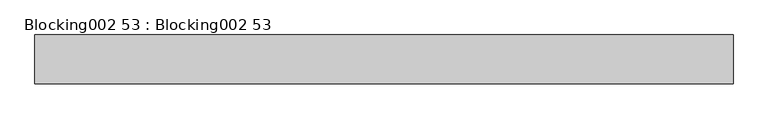
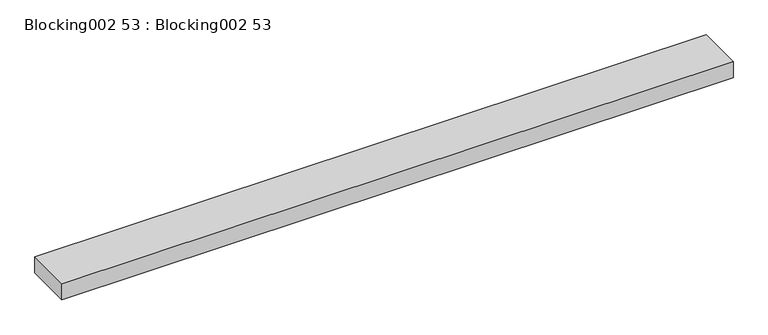
"""IFC4 building model written with IfcOpenShell, lengths in millimetres: proxy geometry, Blocking002 53 : Blocking002 53."""

from ifc_helpers import new_model, si_unit, frame, origin, place, context, project, spatial, polyline, outline, extrude, source, transform, mapped, element, save


def blocking002_53_blocking002_53_1438df7c(model_context):
    return source(origin(), model_context, "Body", "SweptSolid", [
        extrude(outline(polyline([(3694.2883192, 10278.0250834), (3694.2883192, 10417.7250834), (5694.2883192, 10417.7250834), (5694.2883192, 10278.0250834), (3694.2883192, 10278.0250834)])), frame((0.0, 0.0, 40671.496), z_axis=(0.0, 0.0, 1.0), x_axis=(1.0, 0.0, 0.0)), (0.0, 0.0, 1.0), 50.8),
    ])


if __name__ == "__main__":
    model = new_model("IFC4")
    model_context = context("Model", 3, world=origin())
    ifc_project = project(units=[si_unit("LENGTHUNIT", "METRE", prefix="MILLI")], contexts=[model_context])
    site = spatial("IfcSite", under=ifc_project)
    building = spatial("IfcBuilding", under=site)
    placement = place(None, origin())
    blocking002_53_blocking002_53_shape = blocking002_53_blocking002_53_1438df7c(model_context)
    element("IfcBuildingElementProxy", 1, Name="Blocking002 53 : Blocking002 53", ObjectType="Blocking002 53 : Blocking002 53", at=placement, inside=building, context=model_context, shape_type="MappedRepresentation", body=[
        mapped(blocking002_53_blocking002_53_shape, transform((0.0, 0.0, 0.0), x_axis=(1.0, 0.0, 0.0), y_axis=(0.0, 1.0, 0.0), z_axis=(0.0, 0.0, 1.0))),
    ])
    save(model, "model.ifc")

# Revit data of these elements
# Type "Blocking002 53 : Blocking002 53"
#   NameOverride = "Blocking002"
# Element 1 (IfcBuildingElementProxy, "Blocking002 53 : Blocking002 53")
#   Materials on its faces: "WOOD BLOCKING AS REQUIRED"
# Materials
#   "WOOD BLOCKING AS REQUIRED": class "Unassigned", colour RGB 166 124 85, transparency 0, Cost = 0
